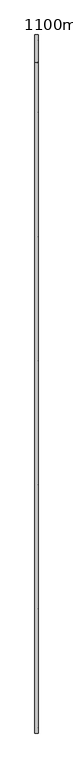
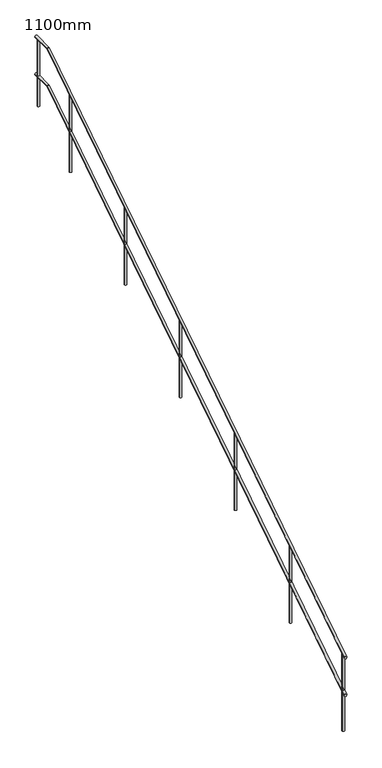
"""IFC4 building model written with IfcOpenShell, lengths in millimetres: railing geometry, 1100mm."""

from ifc_helpers import new_model, si_unit, point, frame, frame_2d, origin, place, context, project, spatial, circle_curve, ellipse_curve, trimmed, segment, composite_curve, outline, extrude, source, transform, mapped, element, save
from ifc_brep_helpers import plane_surface, cylinder_surface, advanced_brep


def railing_1100mm_06c0ee51(model_context):
    return source(origin(), model_context, "Body", "SolidModel", [
        advanced_brep(
        [(19706.6097182, 11187.7630152, 456.1549882), (19736.6097182, 11187.7630152, 456.1549882), (19706.6097182, 17937.7630152, 4635.0), (19736.6097182, 17937.7630152, 4635.0), (19706.6097182, 17672.1776886, 4635.0), (19736.6097182, 17672.1776886, 4635.0)],
        [
            (0, 1, ellipse_curve(frame((19721.6097182, 11187.7630152, 456.1549882), z_axis=(0.0, -1.0, 0.0), x_axis=(0.0, 0.0, -1.0)), 17.8450118, 15.0)),
            (1, 0, ellipse_curve(frame((19721.6097182, 11187.7630152, 456.1549882), z_axis=(0.0, -1.0, 0.0), x_axis=(0.0, 0.0, -1.0)), 17.8450118, 15.0)),
            (2, 3, circle_curve(frame((19721.6097182, 17937.7630152, 4635.0), z_axis=(0.0, 1.0, 0.0), x_axis=(1.0, 0.0, 0.0)), 15.0)),
            (3, 2, circle_curve(frame((19721.6097182, 17937.7630152, 4635.0), z_axis=(0.0, 1.0, 0.0), x_axis=(1.0, 0.0, 0.0)), 15.0)),
            (0, 4),
            (4, 5, ellipse_curve(frame((19721.6097182, 17672.1776886, 4635.0), z_axis=(0.0, -0.9593151294266218, -0.28233753284532276), x_axis=(0.0, 0.282337532845322, -0.9593151294266221)), 15.6361549, 15.0)),
            (5, 1),
            (5, 4, ellipse_curve(frame((19721.6097182, 17672.1776886, 4635.0), z_axis=(0.0, -0.9593151294266218, -0.28233753284532276), x_axis=(0.0, 0.282337532845322, -0.9593151294266221)), 15.6361549, 15.0)),
            (4, 2),
            (3, 5),
        ],
        [
            plane_surface(frame((19721.6097182, 11187.7630152, 474.0), z_axis=(0.0, -1.0, 0.0), x_axis=(0.0, 0.0, 1.0))),
            plane_surface(frame((19721.6097182, 17937.7630152, 4650.0), z_axis=(0.0, 1.0, 0.0), x_axis=(0.0, 0.0, 1.0))),
            cylinder_surface(frame((19721.6097182, 11195.8885352, 461.3914345), z_axis=(0.0, -0.8405710350936326, -0.5417013337270078), x_axis=(1.0, 0.0, 0.0)), 15.0),
            cylinder_surface(frame((19721.6097182, 17667.7630152, 4635.0), z_axis=(0.0, -1.0, 0.0), x_axis=(1.0, 0.0, 0.0)), 15.0),
        ],
        [
            (0, [[1, 2]]),
            (1, [[3, 4]]),
            (2, [[-1, 5, 6, 7]]),
            (2, [[-2, -7, 8, -5]]),
            (3, [[-6, 9, -4, 10]]),
            (3, [[-8, -10, -3, -9]]),
        ],
    ),
        advanced_brep(
        [(19706.6097182, 11187.7630152, 956.1549882), (19736.6097182, 11187.7630152, 956.1549882), (19706.6097182, 17672.1776886, 5135.0), (19736.6097182, 17672.1776886, 5135.0), (19706.6097182, 17937.7630152, 5135.0), (19736.6097182, 17937.7630152, 5135.0)],
        [
            (0, 1, ellipse_curve(frame((19721.6097182, 11187.7630152, 956.1549882), z_axis=(0.0, -1.0, 0.0), x_axis=(0.0, 0.0, -1.0)), 17.8450118, 15.0)),
            (1, 0, ellipse_curve(frame((19721.6097182, 11187.7630152, 956.1549882), z_axis=(0.0, -1.0, 0.0), x_axis=(0.0, 0.0, -1.0)), 17.8450118, 15.0)),
            (0, 2),
            (2, 3, ellipse_curve(frame((19721.6097182, 17672.1776886, 5135.0), z_axis=(0.0, -0.9593151294266218, -0.28233753284532276), x_axis=(0.0, 0.282337532845322, -0.9593151294266221)), 15.6361549, 15.0)),
            (3, 1),
            (3, 2, ellipse_curve(frame((19721.6097182, 17672.1776886, 5135.0), z_axis=(0.0, -0.9593151294266218, -0.28233753284532276), x_axis=(0.0, 0.282337532845322, -0.9593151294266221)), 15.6361549, 15.0)),
            (4, 5, circle_curve(frame((19721.6097182, 17937.7630152, 5135.0), z_axis=(0.0, 1.0, 0.0), x_axis=(1.0, 0.0, 0.0)), 15.0)),
            (5, 4, circle_curve(frame((19721.6097182, 17937.7630152, 5135.0), z_axis=(0.0, 1.0, 0.0), x_axis=(1.0, 0.0, 0.0)), 15.0)),
            (2, 4),
            (5, 3),
        ],
        [
            plane_surface(frame((19721.6097182, 11187.7630152, 974.0), z_axis=(0.0, -1.0, 0.0), x_axis=(0.0, 0.0, 1.0))),
            cylinder_surface(frame((19721.6097182, 11195.8885352, 961.3914345), z_axis=(0.0, -0.8405710350936326, -0.5417013337270078), x_axis=(1.0, 0.0, 0.0)), 15.0),
            plane_surface(frame((19721.6097182, 17937.7630152, 5150.0), z_axis=(0.0, 1.0, 0.0), x_axis=(0.0, 0.0, 1.0))),
            cylinder_surface(frame((19721.6097182, 17667.7630152, 5135.0), z_axis=(0.0, -1.0, 0.0), x_axis=(1.0, 0.0, 0.0)), 15.0),
        ],
        [
            (0, [[1, 2]]),
            (1, [[-1, 3, 4, 5]]),
            (1, [[-2, -5, 6, -3]]),
            (2, [[7, 8]]),
            (3, [[-4, 9, -8, 10]]),
            (3, [[-6, -10, -7, -9]]),
        ],
    ),
        extrude(outline(composite_curve([segment(trimmed(circle_curve(frame_2d((19721.6097182, 17187.7630152)), 15.0), [point((19736.6097182, 17187.7630152))], [point((19706.6097182, 17187.7630152))], False, "CARTESIAN"), True, "CONTINUOUS"), segment(trimmed(circle_curve(frame_2d((19721.6097182, 17187.7630152)), 15.0), [point((19706.6097182, 17187.7630152))], [point((19736.6097182, 17187.7630152))], False, "CARTESIAN"), True, "CONTINUOUS")], self_intersect=False)), frame((0.0, 0.0, 3790.4451685), z_axis=(0.0, 0.0, 1.0), x_axis=(1.0, 0.0, 0.0)), (0.0, 0.0, 1.0), 1020.2214982),
        extrude(outline(composite_curve([segment(trimmed(circle_curve(frame_2d((19721.6097182, 15987.7630152)), 15.0), [point((19736.6097182, 15987.7630152))], [point((19706.6097182, 15987.7630152))], False, "CARTESIAN"), True, "CONTINUOUS"), segment(trimmed(circle_curve(frame_2d((19721.6097182, 15987.7630152)), 15.0), [point((19706.6097182, 15987.7630152))], [point((19736.6097182, 15987.7630152))], False, "CARTESIAN"), True, "CONTINUOUS")], self_intersect=False)), frame((0.0, 0.0, 3017.1118351), z_axis=(0.0, 0.0, 1.0), x_axis=(1.0, 0.0, 0.0)), (0.0, 0.0, 1.0), 1020.2214982),
        extrude(outline(composite_curve([segment(trimmed(circle_curve(frame_2d((19721.6097182, 14787.7630152)), 15.0), [point((19736.6097182, 14787.7630152))], [point((19706.6097182, 14787.7630152))], False, "CARTESIAN"), True, "CONTINUOUS"), segment(trimmed(circle_curve(frame_2d((19721.6097182, 14787.7630152)), 15.0), [point((19706.6097182, 14787.7630152))], [point((19736.6097182, 14787.7630152))], False, "CARTESIAN"), True, "CONTINUOUS")], self_intersect=False)), frame((0.0, 0.0, 2243.7785018), z_axis=(0.0, 0.0, 1.0), x_axis=(1.0, 0.0, 0.0)), (0.0, 0.0, 1.0), 1020.2214982),
        extrude(outline(composite_curve([segment(trimmed(circle_curve(frame_2d((19721.6097182, 13587.7630152)), 15.0), [point((19736.6097182, 13587.7630152))], [point((19706.6097182, 13587.7630152))], False, "CARTESIAN"), True, "CONTINUOUS"), segment(trimmed(circle_curve(frame_2d((19721.6097182, 13587.7630152)), 15.0), [point((19706.6097182, 13587.7630152))], [point((19736.6097182, 13587.7630152))], False, "CARTESIAN"), True, "CONTINUOUS")], self_intersect=False)), frame((0.0, 0.0, 1470.4451685), z_axis=(0.0, 0.0, 1.0), x_axis=(1.0, 0.0, 0.0)), (0.0, 0.0, 1.0), 1020.2214982),
        extrude(outline(composite_curve([segment(trimmed(circle_curve(frame_2d((19721.6097182, 12387.7630152)), 15.0), [point((19736.6097182, 12387.7630152))], [point((19706.6097182, 12387.7630152))], False, "CARTESIAN"), True, "CONTINUOUS"), segment(trimmed(circle_curve(frame_2d((19721.6097182, 12387.7630152)), 15.0), [point((19706.6097182, 12387.7630152))], [point((19736.6097182, 12387.7630152))], False, "CARTESIAN"), True, "CONTINUOUS")], self_intersect=False)), frame((0.0, 0.0, 697.1118351), z_axis=(0.0, 0.0, 1.0), x_axis=(1.0, 0.0, 0.0)), (0.0, 0.0, 1.0), 1020.2214982),
        extrude(outline(composite_curve([segment(trimmed(circle_curve(frame_2d((19721.6097182, 17887.7630152)), 15.0), [point((19736.6097182, 17887.7630152))], [point((19706.6097182, 17887.7630152))], False, "CARTESIAN"), True, "CONTINUOUS"), segment(trimmed(circle_curve(frame_2d((19721.6097182, 17887.7630152)), 15.0), [point((19706.6097182, 17887.7630152))], [point((19736.6097182, 17887.7630152))], False, "CARTESIAN"), True, "CONTINUOUS")], self_intersect=False)), frame((0.0, 0.0, 4241.5562796), z_axis=(0.0, 0.0, 1.0), x_axis=(1.0, 0.0, 0.0)), (0.0, 0.0, 1.0), 878.4437204),
        extrude(outline(composite_curve([segment(trimmed(circle_curve(frame_2d((19721.6097182, 11237.7630152)), 15.0), [point((19736.6097182, 11237.7630152))], [point((19706.6097182, 11237.7630152))], False, "CARTESIAN"), True, "CONTINUOUS"), segment(trimmed(circle_curve(frame_2d((19721.6097182, 11237.7630152)), 15.0), [point((19706.6097182, 11237.7630152))], [point((19736.6097182, 11237.7630152))], False, "CARTESIAN"), True, "CONTINUOUS")], self_intersect=False)), frame((0.0, 0.0, -43.999276), z_axis=(0.0, 0.0, 1.0), x_axis=(1.0, 0.0, 0.0)), (0.0, 0.0, 1.0), 1020.2214982),
    ])


if __name__ == "__main__":
    model = new_model("IFC4")
    model_context = context("Model", 3, world=origin())
    ifc_project = project(units=[si_unit("LENGTHUNIT", "METRE", prefix="MILLI")], contexts=[model_context])
    site = spatial("IfcSite", under=ifc_project)
    building = spatial("IfcBuilding", under=site)
    placement = place(None, origin())
    railing_1100mm_shape = railing_1100mm_06c0ee51(model_context)
    element("IfcRailing", 1, ObjectType="1100mm", at=placement, inside=building, context=model_context, shape_type="MappedRepresentation", body=[
        mapped(railing_1100mm_shape, transform((0.0, 0.0, 0.0), x_axis=(1.0, 0.0, 0.0), y_axis=(0.0, 1.0, 0.0), z_axis=(0.0, 0.0, 1.0))),
    ])
    save(model, "model.ifc")
